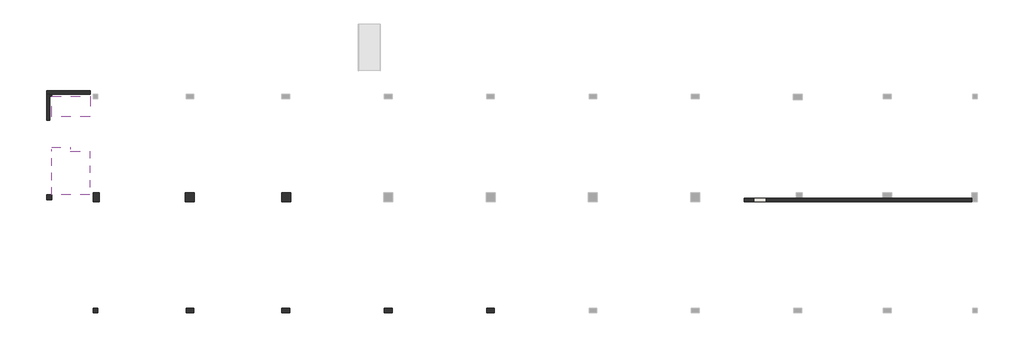
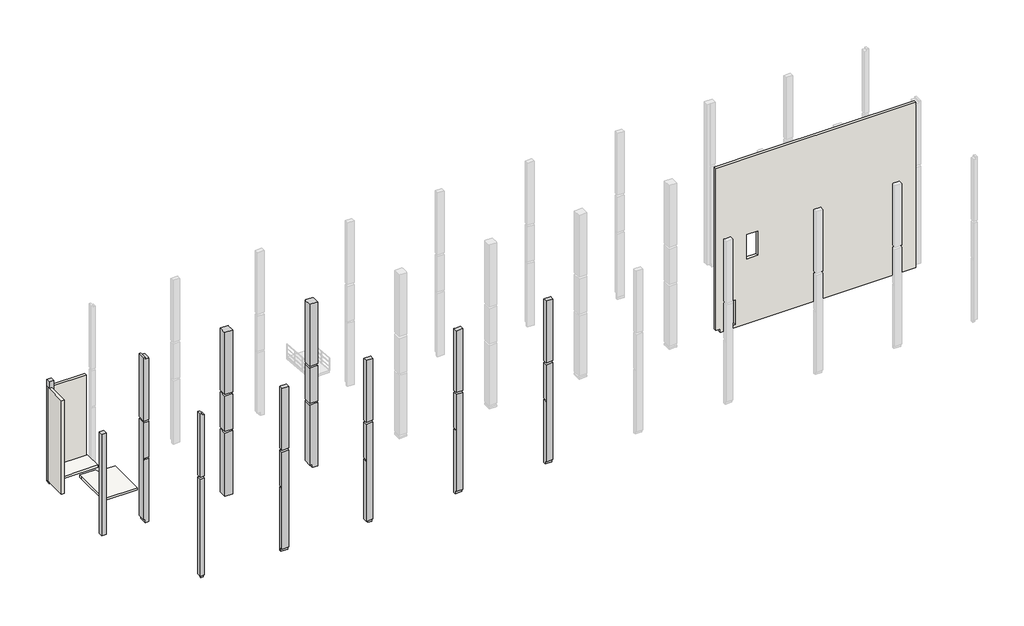
# One storey, part 1 of 3: 10 columns, 3 walls, 2 slabs.
# Revit data of these elements (continued)
# Type "H_FL_AR_S17_RC Slab T200_SS1" (continued)
#   H_WM Code_3 = "A04AQ012-00001 |  | M2 | Finishing Work | Roof Work | PE Sheet (Vapor Barrier) |  | THK=(  )mm |  | A04AQ012-00001 Finishing Work Roof Work PE Sheet (Vapor Barrier)         | Mesh Size=DIA( #8 )mm x ( 150 )mm x (150  )mm"
#   H_WM Code_4 = "A04AQ089-00001 |  | M3 | Finishing Work | Roof Work | Protective Concrete w/ Steel Trowel Finish |  |  |  | A04AQ089-00001 Finishing Work Roof Work Protective Concrete w/ Steel Trowel Finish         | Protective Concrete w/ Steel Trowel Finish (Slope 1%)"
#   H_Rebar ratio = 0.1
#   Function = 1
#   Layers, outside or top first: 200 mm "00_Concrete_Reinf. Conc." (function 1)
# Type "H_WA_AR_B02_Int Wall_RC T250_W2"
#   Type Comments = "CV-AG"
#   Type Mark = "W2"
#   H_Q'ty Cal Type Tag = "WA-Q1"
#   H_WM Code_1 = "A03AF032-00022 |  | M3 | Concrete Work | Superstructure Work | Structural Concrete | Cement Type-1 | 25MPa ≤ F'c (Cylinder Strength) < 30MPa |  |  |  |  | A03AF032-00022 Concrete Work Superstructure Work Structural Concrete  Cement Type-1 25MPa ≤ F'c (Cylinder Strength) < 30MPa      |"
#   H_WM Code_2 = "A03AD037-00002 |  | TON | Concrete Work | Substructure Work | Rebar Work | Deformed Bar (Non-Coat.) | 400MPa<Fy≤470MPa |  |  |  |  | A03AD037-00002 Concrete Work Substructure Work Rebar Work Deformed Bar (Non-Coat.)  400MPa<Fy≤470MPa      |"
#   H_WM Code_3 = "A03AD036-00001 |  | M2 | Concrete Work | Substructure Work | Form Work (1 time in use) | Flat Form | Dressed Lumber, Plywood or Steel Form(Wood Planks are not Allowed) incl. Chamfer |  |  |  | A03AD036-00001 Concrete Work Substructure Work Form Work (1 time in use) Flat Form     Dressed Lumber, Plywood or Steel Form(Wood Planks are not Allowed) incl. Chamfer   |"
#   H_WM Code_4 = "A04AM077-00001 |  | M2 | Finishing Work | Painting Work | External Wall Painting | Acrylic Emulsion Paint |  |  |  |  | A04AM077-00001 Finishing Work Painting Work External Wall Painting Acrylic Emulsion Paint        |"
#   H_Rebar ratio = 0.12
#   Layers, outside or top first: 250 mm "00_Concrete_Reinf. Conc." (function 1)
# Type "H_WA_AR_B02_Ext Wall_RC T250_W1_Stair"
#   Type Comments = "CV-AG"
#   Type Mark = "W1"
#   H_Q'ty Cal Type Tag = "SF-Q5"
#   H_WM Code_1 = "A03AD032-00022 |  | M3 | Concrete Work | Substructure Work | Structural Concrete | Cement Type-1 | 25MPa ≤ F'c (Cylinder Strength) < 30MPa |  |  |  |  | A03AD032-00022 Concrete Work Substructure Work Structural Concrete  Cement Type-1 25MPa ≤ F'c (Cylinder Strength) < 30MPa      |  F'c (Cylinder Strength) = 24MPa"
#   H_WM Code_2 = "A03AD037-00002 |  | TON | Concrete Work | Substructure Work | Rebar Work | Deformed Bar (Non-Coat.) | 400MPa<Fy≤470MPa |  |  |  |  | A03AD037-00002 Concrete Work Substructure Work Rebar Work Deformed Bar (Non-Coat.)  400MPa<Fy≤470MPa      | ASTM A615 GRADE 60 (Fy=420MPa)"
#   H_WM Code_3 = "A03AD035-00001 |  | M2 | Concrete Work | Substructure Work | Form Work (3 times in use) | Flat Form | Dressed Lumber, Plywood or Steel Form(Wood Planks are not Allowed) incl. Chamfer |  |  |  | A03AD035-00001 Concrete Work Substructure Work Form Work (3 times in use) Flat Form     Dressed Lumber, Plywood or Steel Form(Wood Planks are not Allowed) incl. Chamfer   |"
#   H_WM Code_4 = "A03AH056-00001 |  | M2 | Concrete Work | Concrete Protective Coating (U/G) | Bitumen/Bituminous/Asphalt Coating |  |  | A03AH056-00001 Concrete Work Concrete Protective Coating (U/G) Bitumen/Bituminous/Asphalt Coating         |"
#   H_WM Code_5 = "A03AD047-00004 |  | M2 | Concrete Work | Substructure Work | Insulation under Ground Floor | Extruded Polystyrene Insulation Board |  | 100mm≤THK | THK=(  )mm |  | A03AD047-00004 Concrete Work Substructure Work Insulation under Ground Floor Extruded Polystyrene Insulation Board       100mm≤THK |"
#   H_WM Code_6 = "A01ZZ001-00012 |  | M3 | Earth Work | - | Excavation | Soil, Mech. |  | Manual Excavation Above GWL |  |  |  | A01ZZ001-00012 Earth Work - Excavation Soil, Mech.      Manual Excavation Above GWL  | Above GWL"
#   H_WM Code_7 = "A01ZZ001-00013 |  | M3 | Earth Work | - | Excavation | Soil, Mech. |  | Manual Excavation Below GWL |  |  |  | A01ZZ001-00013 Earth Work - Excavation Soil, Mech.      Manual Excavation Below GWL  | Below GWL"
#   H_WM Code_8 = "A01ZZ003-00001 |  | M3 | Earth Work | - | Backfill | Re-use, Soil |  |  |  | Compaction=(  )% |  | A01ZZ003-00001 Earth Work - Backfill Re-use, Soil        | Compaction=( 95 )%"
#   H_WM Code_9 = "A01ZZ004-00001 |  | M3 | Earth Work | - | Disposal | Soil |  |  |  | Disposal Distance=Appx. (  )km from Site |  | A01ZZ004-00001 Earth Work - Disposal Soil        | Disposal Distance=Appx. (20 )km from Site"
#   H_WM Code_10 = "A03AH056-00001 |  | M2 | Concrete Work | Concrete Protective Coating (U/G) | Bitumen/Bituminous/Asphalt Coating |  |  | A03AH056-00001 Concrete Work Concrete Protective Coating (U/G) Bitumen/Bituminous/Asphalt Coating         | *기초바닥 Protection 은 Lean에 적용"
#   H_Rebar ratio = 0.12
#   Layers, outside or top first: 0 mm no material (function 100); 0 mm no material (function 100); 250 mm "00_Concrete_Reinf. Conc." (function 1); 0 mm no material (function 100); 0 mm no material (function 100); 0 mm no material (function 100)
# Elements 1, 2, 3 (IfcColumn, "RC_Column_Rectangular : H_SC_AR_S15_AG_W700xL700_C1")
#   Comments = ""
#   hec_material3 = none
#   hec_material2 = none
#   hec_material1 = none
#   Structural Material = 00_Concrete_Reinf. Conc.
#   Phase Created = New Construction
#   Materials on its faces: "00_Concrete_Reinf. Conc."
# Elements 4, 5, 6, 7, 8 (IfcColumn, "RC_Column_Rectangular : H_SC_AR_S15_AG_W600xL600_C2")
#   Comments = ""
#   hec_material3 = none
#   hec_material2 = none
#   hec_material1 = none
#   Structural Material = 00_Concrete_Reinf. Conc.
#   Phase Created = New Construction
#   Materials on its faces: "00_Concrete_Reinf. Conc."
# Elements 9, 10 (IfcColumn, "RC_Column_Rectangular : H_SC_AR_S15_AG_W400xL400_C3")
#   Comments = ""
#   hec_material3 = none
#   hec_material2 = none
#   hec_material1 = none
#   Structural Material = 00_Concrete_Reinf. Conc.
#   Phase Created = New Construction
#   Materials on its faces: "00_Concrete_Reinf. Conc."
# Element 11 (IfcSlab, "H_FL_AR_S17_RC Slab T200_SS1")
#   Comments = ""
#   TMP_Element Name = "SS2"
#   built-in parameter 1001955 = 3.14159 (stored number, unit not read)
#   Height Offset From Level = 1522.941 mm
#   built-in parameter 1001954 = 1
#   Phase Created = New Construction
#   Materials on its faces: "00_Concrete_Reinf. Conc."
# Element 12 (IfcSlab, "H_FL_AR_S17_RC Slab T200_SS1")
#   Comments = ""
#   TMP_Element Name = "SS2"
#   built-in parameter 1001955 = 3.14159 (stored number, unit not read)
#   Height Offset From Level = 3090 mm
#   built-in parameter 1001954 = 1
#   Phase Created = New Construction
#   Materials on its faces: "00_Concrete_Reinf. Conc."
# Element 13 (IfcWall, "H_WA_AR_B02_Int Wall_RC T250_W2")
#   Comments = ""
#   Top Offset = 0 mm
#   Base Offset = 0 mm
#   wall height = 15560 mm
#   Phase Created = New Construction
#   Base Constraint = G.L
#   Top Constraint = TOF3
#   Materials on its faces: "00_Concrete_Reinf. Conc."
# Element 14 (IfcWall, "H_WA_AR_B02_Ext Wall_RC T250_W1_Stair")
#   Comments = ""
#   built-in parameter 1001111 = 130 mm
#   Top Offset = 150 mm
#   Base Offset = 130 mm
#   Unconnected Height = 8820 mm
#   wall height = 8820 mm
#   Phase Created = New Construction
#   Base Constraint = G.L
#   Materials on its faces: "Default Wall", "00_Concrete_Reinf. Conc."
# Element 15 (IfcWall, "H_WA_AR_B02_Ext Wall_RC T250_W1_Stair")
#   Comments = ""
#   built-in parameter 1001111 = 130 mm
#   Top Offset = 150 mm
#   Base Offset = 130 mm
#   Unconnected Height = 8820 mm
#   wall height = 8820 mm
#   Phase Created = New Construction
#   Base Constraint = G.L
#   Materials on its faces: "00_Concrete_Reinf. Conc.", "Default Wall"
# Materials
#   "00_Concrete_Reinf. Conc.": class "Concrete", colour RGB 176 176 176, transparency 0, Description = "Reinf. Conc.", Cost = 0, Image = Concrete.Cast-In-Place.Flat.Polished.Grey.jpg
#   "Default Wall": class "Miscellaneous", colour RGB 80 80 80, transparency 0
